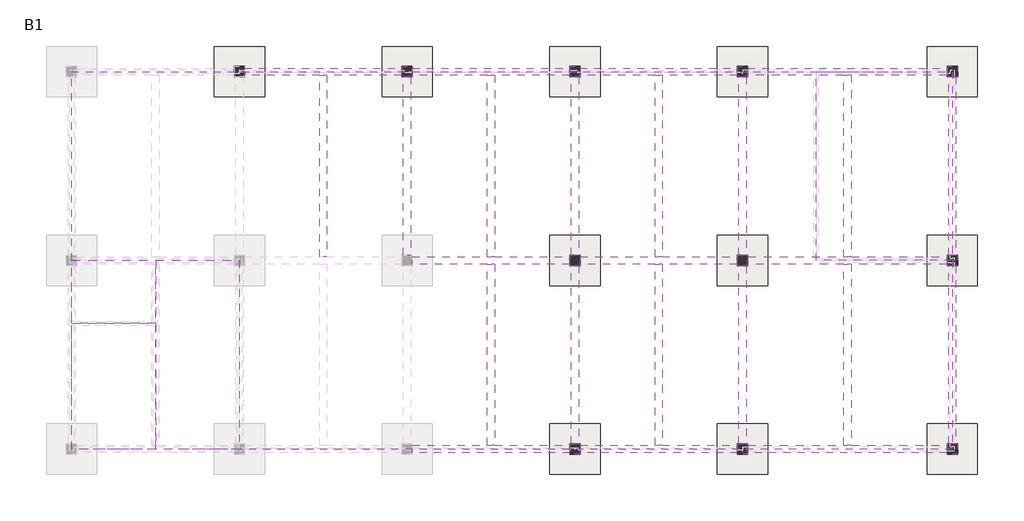
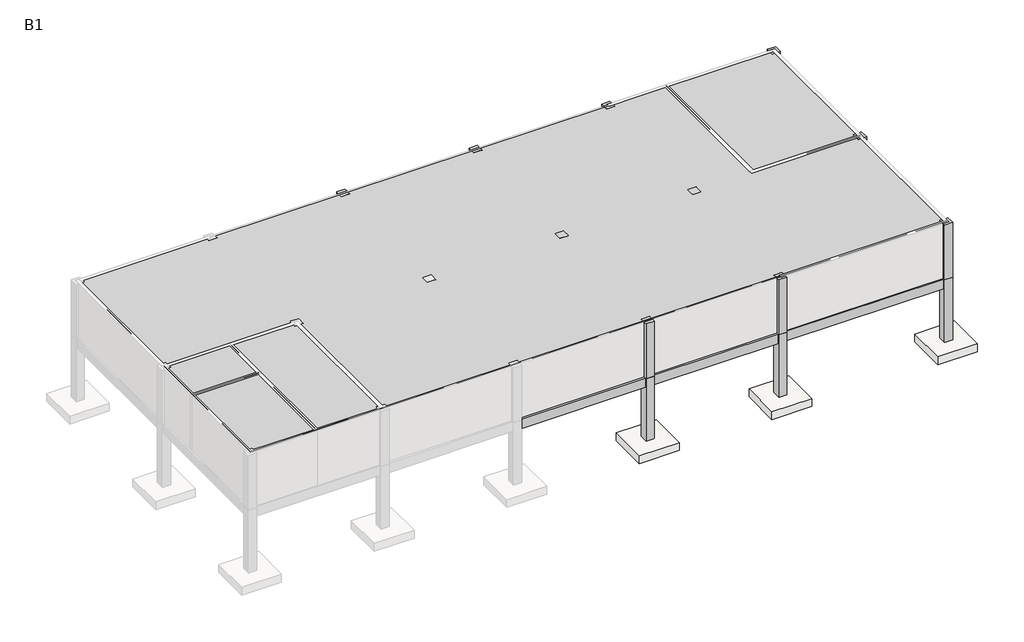
# One storey, part 2 of 2: 24 beams, 21 columns, 11 slabs, 5 proxies.
# Revit data of these elements (continued)
# Element 27 (IfcBuildingElementProxy, "Space Planning Box_hec : Space Planning Box_hec") (continued)
#   Interior Finish = "IW5..N/A..N/A,,WK3..N/A,,FL2..N/A,,N/A..N/A"
#   Exterior Finish = "N/A..N/A,,EW2..N/A..N/A"
#   Department = "AR"
#   ceiling height = 0
#   Width = 4000 mm
#   Program Area = 0.00 m²
#   Length = 9000 mm
#   Height = 3500 mm
#   Area = 36.00 m²
#   Fill Color = Cyan
#   Phase Created = New Construction
#   Materials on its faces: "Cyan"
# Element 28 (IfcBuildingElementProxy, "Space Planning Box_hec : Space Planning Box_hec")
#   Room Name = "Elevator"
#   Interior Finish = "N/A..N/A..N/A,,N/A..N/A,,,,CL3..N/A"
#   Exterior Finish = "N/A..N/A,,EW2..N/A..N/A"
#   Department = "AR"
#   ceiling height = 0
#   Width = 4000 mm
#   Program Area = 0.00 m²
#   Length = 3000 mm
#   Height = 3500 mm
#   Area = 12.00 m²
#   Fill Color = Cyan
#   Phase Created = New Construction
#   Materials on its faces: "Cyan"
# Element 29 (IfcBuildingElementProxy, "Space Planning Box_hec : Space Planning Box_hec")
#   Room Name = "Stairway"
#   Interior Finish = "IW5..N/A..N/A,,WK3..N/A,,FL2..N/A,,CL1..N/A"
#   Exterior Finish = "N/A..N/A,,EW2..N/A..N/A"
#   Department = "PATHV1"
#   ceiling height = 0
#   Width = 4000 mm
#   Program Area = 36.00 m²
#   Length = 6000 mm
#   Height = 3500 mm
#   Area = 24.00 m²
#   Fill Color = Green
#   Phase Created = New Construction
#   Materials on its faces: "Green"
# Elements 30, 31, 32, 33, 34, 35, 36, 37, 38, 39, 40, 41, 42, 43, 44, 45, 46, 47, 48, 49, 50 (IfcColumn, "Concrete-Rectangular-Column : CL111_500x500")
#   Comments = ""
#   hec_material3 = none
#   hec_material2 = none
#   hec_material1 = none
#   Structural Material = 콘크리트 - 현장타설 콘크리트
#   Phase Created = New Construction
#   Materials on its faces: "콘크리트 - 현장타설 콘크리트"
# Elements 51, 52, 53, 54, 55, 56, 57, 58, 59, 60, 61 (IfcSlab, "FT112-Footing-Rectangular : FT112_2400x2400x500")
#   Comments = ""
#   hec_material3 = none
#   hec_material2 = none
#   hec_material1 = none
#   Structural Material = 콘크리트 - 현장타설 콘크리트
#   Phase Created = New Construction
#   Materials on its faces: "콘크리트 - 현장타설 콘크리트"
# Materials
#   "콘크리트 - 현장타설 콘크리트": class "콘크리트", colour RGB 192 192 192, transparency 0
#   "Cyan": class "Generic", colour RGB 0 255 255, transparency 0.2, Cost = 0
#   "A03AE056-00001_Bitumen/Bituminous/Asphalt Coating": class "Generic", colour RGB 17 17 17, transparency 0, Description = "Damp-proofing", W00) Work Master Code = "A03AE056-00001", W01) Work Master_Lv1 = "Concrete Work", W02) Work Master_Lv2 = "Concrete Protective Coating (U/G)", W03) Work Master_Spec.1 = "Bitumen/Bituminous/Asphalt Coating", Cost = 0
#   "A03AC035-00001_Form Work (3 times in use)_Flat": class "Wood", colour RGB 149 120 74, transparency 0, Description = "Plywood", W00) Work Master Code = "A03AC035-00001", W01) Work Master_Lv1 = "Concrete Work", W02) Work Master_Lv2 = "Substructure Work", W03) Work Master_Spec.1 = "Form Work (3 times in use)", W04) Work Master_Spec.2 = "Flat Form", W05) Work Master_Spec.3 = "Dressed Lumber, Plywood or Steel Form(Wood Planks are not Allowed) incl. Chamfer", Cost = 0
#   "A03AC032-00007_Structural Concrete_Type1_25MPa-30Mpa": class "Concrete", colour RGB 176 176 176, transparency 0, Keynote = "09910.A1", Description = "Reinf. Conc.", W00) Work Master Code = "A03AC032-00007", W01) Work Master_Lv1 = "Concrete Work", W02) Work Master_Lv2 = "Substructure Work", W03) Work Master_Spec.1 = "Structural Concrete", W04) Work Master_Spec.2 = "Cement Type-1", W05) Work Master_Spec.3 = "25MPa < F'c (Cylinder Strength) ≤ 30MPa", Cost = 0
#   "Orange": class "Generic", colour RGB 255 165 0, transparency 0.2, Cost = 0
#   "Green": class "Generic", colour RGB 0 128 0, transparency 0.2, Cost = 0
# Room at (84209.652, 177423.861) mm, phase "New Construction", upper offset 3500 mm, lower offset 0 mm
#   Department = "EL"
#   Base Finish = ""
#   Ceiling Finish = "CL2"
#   Wall Finish = "IW2"
#   Floor Finish = "FL7"
#   Number = "0.0"
#   Name = "Battery Room"
#   Interior Finish = "IW2..N/A..N/A,,N/A..N/A,,FL7..N/A,,CL2..N/A"
#   Exterior Finish = "N/A..N/A,,EW2..N/A..N/A"
# Room at (51459.652, 168423.861) mm, phase "New Construction", upper offset 3500 mm, lower offset 0 mm
#   Department = "AR"
#   Base Finish = "WK3"
#   Ceiling Finish = ""
#   Wall Finish = "IW5"
#   Floor Finish = "FL2"
#   Number = "0.1"
#   Name = "Lobby"
#   Interior Finish = "IW5..N/A..N/A,,WK3..N/A,,FL2..N/A,,N/A..N/A"
#   Exterior Finish = "N/A..N/A,,EW2..N/A..N/A"
# Room at (66459.652, 172923.861) mm, phase "New Construction", upper offset 3500 mm, lower offset 0 mm
#   Department = "EL"
#   Base Finish = "WK1"
#   Ceiling Finish = "CL1"
#   Wall Finish = "IW5,IW2"
#   Floor Finish = "FL1"
#   Number = "0.2"
#   Name = "Cable Room"
#   Interior Finish = "IW5..IW2..N/A,,WK1..N/A,,FL1..N/A,,CL1..N/A"
#   Exterior Finish = "N/A..N/A,,EW1..EW2..N/A"
# Room at (47459.652, 166923.861) mm, phase "New Construction", upper offset 3500 mm, lower offset 0 mm
#   Department = "PATHV1"
#   Base Finish = "WK3"
#   Ceiling Finish = "CL1"
#   Wall Finish = "IW5"
#   Floor Finish = "FL2"
#   Number = "0.3"
#   Name = "Stairway"
#   Interior Finish = "IW5..N/A..N/A,,WK3..N/A,,FL2..N/A,,CL1..N/A"
#   Exterior Finish = "N/A..N/A,,EW2..N/A..N/A"
# Room at (47459.652, 171423.861) mm, phase "New Construction", upper offset 3500 mm, lower offset 0 mm
#   Department = "AR"
#   Base Finish = ""
#   Ceiling Finish = "CL3"
#   Wall Finish = ""
#   Floor Finish = ""
#   Number = "0.4"
#   Name = "Elevator"
#   Interior Finish = "N/A..N/A..N/A,,N/A..N/A,,,,CL3..N/A"
#   Exterior Finish = "N/A..N/A,,EW2..N/A..N/A"
